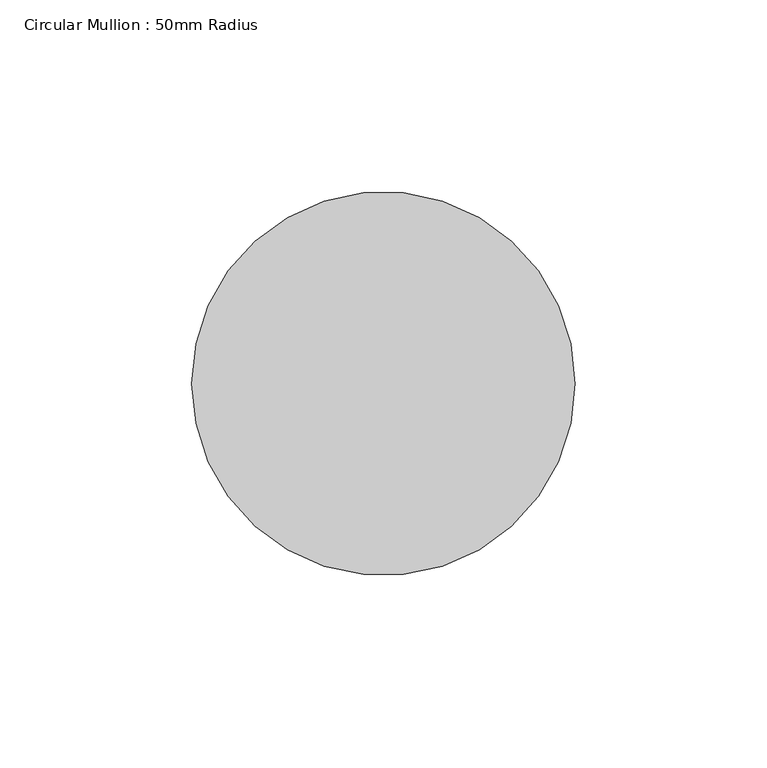
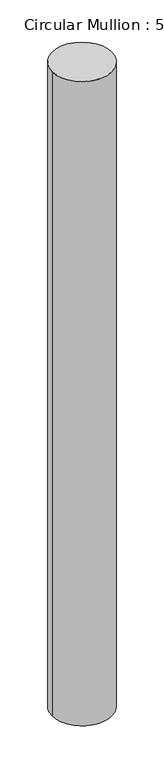
"""IFC4 building model written with IfcOpenShell, lengths in millimetres: member geometry, Circular Mullion : 50mm Radius."""

import ifcopenshell
import ifcopenshell.guid

model = None  # the IFC model being written
_history = None  # IfcOwnerHistory: only IFC2X3 demands one
_inside = {}  # id of a spatial element -> (the spatial element, [elements in it])
_under = {}  # id of a project, library or spatial element -> (it, [spatial elements below it])
_declared = {}  # id of a project -> (the project, [libraries it declares])
_typed = {}  # id of a type object -> (the type object, [elements of that type])
_made_of = {}  # id of a material, layer set ... -> (it, [elements and type objects made of it])


def new_model(schema):
    """Start an empty IFC model of exactly this schema.

    Asked for "IFC4X3", IfcOpenShell would pick the latest addendum, in which some entities
    have other attributes; the version numbers below select the first issue.
    IFC2X3 requires an IfcOwnerHistory on every rooted entity: one is made here for all.
    """
    global model, _history
    if schema == "IFC4X3":
        model = ifcopenshell.file(schema_version=(4, 3, 0, 0))
    else:
        model = ifcopenshell.file(schema=schema)
    _inside.clear()
    _under.clear()
    _declared.clear()
    _typed.clear()
    _made_of.clear()
    _history = None
    if model.schema == "IFC2X3":
        org = make("IfcOrganization", Name="unknown")
        user = make(
            "IfcPersonAndOrganization",
            ThePerson=make("IfcPerson", FamilyName="unknown"),
            TheOrganization=org,
        )
        app = make(
            "IfcApplication",
            ApplicationDeveloper=org,
            Version="unknown",
            ApplicationFullName="unknown",
            ApplicationIdentifier="unknown",
        )
        _history = make(
            "IfcOwnerHistory",
            OwningUser=user,
            OwningApplication=app,
            ChangeAction="ADDED",
            CreationDate=0,
        )
    return model


def make(cls, **values):
    """One entity of the class cls with the attributes given. An attribute that is None is left unset."""
    return model.create_entity(
        cls, **{name: value for name, value in values.items() if value is not None}
    )


def rooted(cls, **values):
    """An entity with a GlobalId (a new one), such as an element, a storey or a relation."""
    return make(cls, GlobalId=ifcopenshell.guid.new(), OwnerHistory=_history, **values)


def si_unit(unit_type, name, prefix=None):
    """IfcSIUnit, for example si_unit("LENGTHUNIT", "METRE", prefix="MILLI")."""
    return make("IfcSIUnit", UnitType=unit_type, Prefix=prefix, Name=name)


def assignment(units):
    """IfcUnitAssignment: the units of a project."""
    return None if units is None else make("IfcUnitAssignment", Units=units)


def point(xyz):
    """IfcCartesianPoint."""
    return None if xyz is None else make("IfcCartesianPoint", Coordinates=xyz)


def direction(xyz):
    """IfcDirection."""
    return None if xyz is None else make("IfcDirection", DirectionRatios=xyz)


def frame(location, z_axis=None, x_axis=None):
    """IfcAxis2Placement3D, a coordinate frame: its origin and axes. An axis left out is left unset."""
    return make(
        "IfcAxis2Placement3D",
        Location=point(location),
        Axis=direction(z_axis),
        RefDirection=direction(x_axis),
    )


def frame_2d(location, x_axis=None):
    """IfcAxis2Placement2D, a coordinate frame in the plane: its origin and x axis."""
    return make(
        "IfcAxis2Placement2D", Location=point(location), RefDirection=direction(x_axis)
    )


def origin():
    """The frame at (0, 0, 0) with its axes left unset."""
    return frame((0.0, 0.0, 0.0))


def origin_2d():
    """The frame at (0, 0) in the plane with its x axis left unset."""
    return frame_2d((0.0, 0.0))


def place(relative_to, where):
    """IfcLocalPlacement: puts the frame where relative to a parent placement (None: the world)."""
    return make(
        "IfcLocalPlacement", PlacementRelTo=relative_to, RelativePlacement=where
    )


def context(
    kind, dimensions, precision=None, world=None, true_north=None, identifier=None
):
    """IfcGeometricRepresentationContext, for example the 3D "Model" context."""
    return make(
        "IfcGeometricRepresentationContext",
        ContextIdentifier=identifier,
        ContextType=kind,
        CoordinateSpaceDimension=dimensions,
        Precision=precision,
        WorldCoordinateSystem=world,
        TrueNorth=true_north,
    )


def project(units=None, contexts=None):
    """IfcProject with its units and contexts."""
    return rooted(
        "IfcProject",
        Name="project",
        RepresentationContexts=contexts,
        UnitsInContext=assignment(units),
    )


def spatial(cls, under=None, at=None, **own):
    """A site, building, storey or space (cls), placed at a placement, below another one or the project."""
    s = rooted(cls, ObjectPlacement=at, **own)
    if under is not None:
        _under.setdefault(under.id(), (under, []))[1].append(s)
    return s


def circle_curve(where, radius):
    """IfcCircle in the frame where."""
    return make("IfcCircle", Position=where, Radius=radius)


def trimmed(basis, trim1, trim2, sense, master):
    """IfcTrimmedCurve: the piece of a basis curve between two trims."""
    return make(
        "IfcTrimmedCurve",
        BasisCurve=basis,
        Trim1=trim1,
        Trim2=trim2,
        SenseAgreement=sense,
        MasterRepresentation=master,
    )


def segment(curve, same_sense, transition):
    """IfcCompositeCurveSegment."""
    return make(
        "IfcCompositeCurveSegment",
        Transition=transition,
        SameSense=same_sense,
        ParentCurve=curve,
    )


def composite_curve(segments, self_intersect=None):
    """IfcCompositeCurve: segments joined end to end."""
    return make("IfcCompositeCurve", Segments=segments, SelfIntersect=self_intersect)


def outline(outer, holes=None, kind="AREA"):
    """IfcArbitraryClosedProfileDef: a profile drawn as a closed curve; with holes, ...WithVoids."""
    if holes is None:
        return make("IfcArbitraryClosedProfileDef", ProfileType=kind, OuterCurve=outer)
    return make(
        "IfcArbitraryProfileDefWithVoids",
        ProfileType=kind,
        OuterCurve=outer,
        InnerCurves=holes,
    )


def extrude(swept, where, along, depth):
    """IfcExtrudedAreaSolid: the profile swept, set in the frame where, extruded along a direction by depth."""
    return make(
        "IfcExtrudedAreaSolid",
        SweptArea=swept,
        Position=where,
        ExtrudedDirection=direction(along),
        Depth=depth,
    )


def shape(context_of_items, identifier, shape_type, items):
    """IfcShapeRepresentation: the items that make up one representation, for example the "Body"."""
    return make(
        "IfcShapeRepresentation",
        ContextOfItems=context_of_items,
        RepresentationIdentifier=identifier,
        RepresentationType=shape_type,
        Items=items,
    )


def source(mapping_origin, context_of_items, identifier, shape_type, items):
    """IfcRepresentationMap: a shape defined once, which mapped items show again and again."""
    return make(
        "IfcRepresentationMap",
        MappingOrigin=mapping_origin,
        MappedRepresentation=shape(context_of_items, identifier, shape_type, items),
    )


def transform(
    local_origin,
    x_axis=None,
    y_axis=None,
    z_axis=None,
    scale=None,
    scale2=None,
    scale3=None,
    uniform=True,
):
    """IfcCartesianTransformationOperator3D, or its non-uniform kind. x_axis, y_axis, z_axis: its Axis1, 2, 3."""
    if uniform:
        return make(
            "IfcCartesianTransformationOperator3D",
            Axis1=direction(x_axis),
            Axis2=direction(y_axis),
            LocalOrigin=point(local_origin),
            Scale=scale,
            Axis3=direction(z_axis),
        )
    return make(
        "IfcCartesianTransformationOperator3DnonUniform",
        Axis1=direction(x_axis),
        Axis2=direction(y_axis),
        LocalOrigin=point(local_origin),
        Scale=scale,
        Axis3=direction(z_axis),
        Scale2=scale2,
        Scale3=scale3,
    )


def mapped(mapping_source, mapping_target):
    """IfcMappedItem: shows the shape of a source again, moved by a transform."""
    return make(
        "IfcMappedItem", MappingSource=mapping_source, MappingTarget=mapping_target
    )


def made_of(thing, what):
    """Note that an element or type object is made of a material, layer set ...; save() writes the relation."""
    if what is not None:
        _made_of.setdefault(what.id(), (what, []))[1].append(thing)
    return thing


def element(
    cls,
    number,
    at=None,
    inside=None,
    cuts=None,
    type_object=None,
    material=None,
    context=None,
    identifier="Body",
    shape_type=None,
    held_by="IfcProductDefinitionShape",
    body=None,
    shapes=None,
    **own,
):
    """One element of the class cls, such as IfcWall. Its Tag is "e" and its number.

    at: its placement. inside: the storey or other place that contains it. cuts: it is an
    opening in that element (IfcRelVoidsElement). A single representation is given by context,
    identifier, shape_type and body (its items); several are given by shapes. held_by: the class
    of the entity that holds the representations. save() writes the other relations.
    """
    e = rooted(cls, Tag="e%d" % number, ObjectPlacement=at, **own)
    if body is not None:
        shapes = [shape(context, identifier, shape_type, body)]
    if shapes is not None:
        e.Representation = make(held_by, Representations=shapes)
    if inside is not None:
        _inside.setdefault(inside.id(), (inside, []))[1].append(e)
    if cuts is not None:
        rooted(
            "IfcRelVoidsElement", RelatingBuildingElement=cuts, RelatedOpeningElement=e
        )
    if type_object is not None:
        _typed.setdefault(type_object.id(), (type_object, []))[1].append(e)
    return made_of(e, material)


def aggregate(whole, parts):
    """IfcRelAggregates: a whole, such as a stair, and the parts it consists of."""
    return rooted("IfcRelAggregates", RelatingObject=whole, RelatedObjects=parts)


def save(model, path):
    """Write the relations noted so far, then the file.

    IfcRelAggregates (storeys below a building ...), IfcRelContainedInSpatialStructure (elements
    in a storey), IfcRelDefinesByType, IfcRelAssociatesMaterial and IfcRelDeclares: one each for
    every whole, place, type object, material and project.
    """
    for whole, parts in _under.values():
        aggregate(whole, parts)
    for where, things in _inside.values():
        rooted(
            "IfcRelContainedInSpatialStructure",
            RelatedElements=things,
            RelatingStructure=where,
        )
    for kind, things in _typed.values():
        rooted("IfcRelDefinesByType", RelatedObjects=things, RelatingType=kind)
    for what, things in _made_of.values():
        rooted("IfcRelAssociatesMaterial", RelatedObjects=things, RelatingMaterial=what)
    for by, libraries in _declared.values():
        rooted("IfcRelDeclares", RelatingContext=by, RelatedDefinitions=libraries)
    model.write(path)


def circular_mullion_50mm_radius_51bf8f36(model_context):
    return source(origin(), model_context, "Body", "SweptSolid", [
        extrude(outline(composite_curve([segment(trimmed(circle_curve(origin_2d(), 50.0), [point((50.0, 0.0))], [point((-50.0, 0.0))], False, "CARTESIAN"), True, "CONTINUOUS"), segment(trimmed(circle_curve(origin_2d(), 50.0), [point((-50.0, 0.0))], [point((50.0, 0.0))], False, "CARTESIAN"), True, "CONTINUOUS")], self_intersect=False)), frame((0.0, 0.0, -1141.7590864), z_axis=(0.0, 0.0, 1.0), x_axis=(1.0, 0.0, 0.0)), (0.0, 0.0, 1.0), 1141.7590864),
    ])


if __name__ == "__main__":
    model = new_model("IFC4")
    model_context = context("Model", 3, world=origin())
    ifc_project = project(units=[si_unit("LENGTHUNIT", "METRE", prefix="MILLI")], contexts=[model_context])
    site = spatial("IfcSite", under=ifc_project)
    building = spatial("IfcBuilding", under=site)
    placement = place(None, origin())
    circular_mullion_50mm_radius_shape = circular_mullion_50mm_radius_51bf8f36(model_context)
    element("IfcMember", 1, ObjectType="Circular Mullion : 50mm Radius", at=placement, inside=building, context=model_context, shape_type="MappedRepresentation", body=[
        mapped(circular_mullion_50mm_radius_shape, transform((0.0, 0.0, 0.0), x_axis=(1.0, 0.0, 0.0), y_axis=(0.0, 1.0, 0.0), z_axis=(0.0, 0.0, 1.0))),
    ])
    save(model, "model.ifc")

# Revit data of these elements
# Type "Circular Mullion : 50mm Radius"
#   built-in parameter 1007350 = 0.164042 (stored number, unit not read)
# Element 1 (IfcMember, "Circular Mullion : 50mm Radius")
#   Materials on its faces: "Aluminium"
# Materials
#   "Aluminium": class "Metal", colour RGB 247 247 247, transparency 0, Description = "Aluminium 6061", Cost = 0
